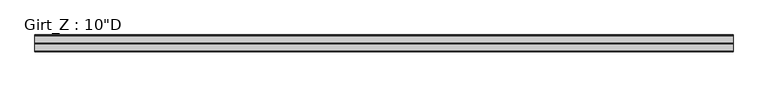
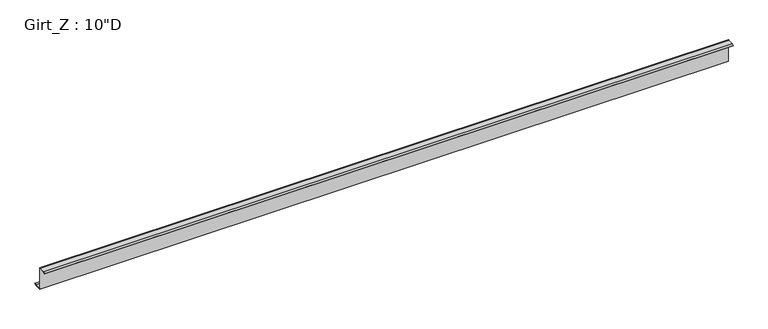
"""IFC4 building model written with IfcOpenShell, lengths in millimetres: beam geometry."""

from ifc_helpers import new_model, si_unit, point, frame, frame_2d, origin, place, context, project, spatial, polyline, circle_curve, trimmed, segment, composite_curve, outline, extrude, source, transform, mapped, element, save


def beam_e7052807(model_context):
    return source(origin(), model_context, "Body", "SweptSolid", [
        extrude(outline(composite_curve([segment(polyline([(-77.9859375, 127.0), (-3.3734375, 127.0)]), True, "CONTINUOUS"), segment(trimmed(circle_curve(frame_2d((-3.3734375, 122.2375)), 4.7625), [point((-3.3734375, 127.0))], [point((1.3890625, 122.2375))], False, "CARTESIAN"), True, "CONTINUOUS"), segment(polyline([(1.3890625, 122.2375), (1.3890625, -122.2389339)]), True, "CONTINUOUS"), segment(trimmed(circle_curve(frame_2d((3.3748024, -122.2389339)), 1.9857399), [point((1.3890625, -122.2389339))], [point((3.2694106, -124.221875))], True, "CARTESIAN"), True, "CONTINUOUS"), segment(polyline([(3.2694106, -124.221875), (83.0404765, -124.221875), (94.4528742, -110.621109), (96.5810415, -112.4068534), (84.3359375, -127.0), (-1.3890625, -127.0), (-1.3890625, 122.2381931)]), True, "CONTINUOUS"), segment(trimmed(circle_curve(frame_2d((-3.3741066, 122.2381931)), 1.9850441), [point((-1.3890625, 122.2381931))], [point((-3.3005807, 124.221875))], True, "CARTESIAN"), True, "CONTINUOUS"), segment(polyline([(-3.3005807, 124.221875), (-76.6904765, 124.221875), (-88.1028742, 110.621109), (-90.2310415, 112.4068534), (-77.9859375, 127.0)]), True, "CONTINUOUS")], self_intersect=False)), frame((-3811.1049, 0.0, 0.0), z_axis=(1.0, 0.0, 0.0), x_axis=(0.0, 1.0, 0.0)), (0.0, 0.0, 1.0), 7692.644),
    ])


if __name__ == "__main__":
    model = new_model("IFC4")
    model_context = context("Model", 3, world=origin())
    ifc_project = project(units=[si_unit("LENGTHUNIT", "METRE", prefix="MILLI")], contexts=[model_context])
    site = spatial("IfcSite", under=ifc_project)
    building = spatial("IfcBuilding", under=site)
    placement = place(None, origin())
    beam_shape = beam_e7052807(model_context)
    element("IfcBeam", 1, ObjectType="Girt_Z : 10\"D", at=placement, inside=building, context=model_context, shape_type="MappedRepresentation", body=[
        mapped(beam_shape, transform((0.0, 0.0, 0.0), x_axis=(1.0, 0.0, 0.0), y_axis=(0.0, 1.0, 0.0), z_axis=(0.0, 0.0, 1.0))),
    ])
    save(model, "model.ifc")

# Revit data of these elements
# Type "Girt_Z : 10\"D"
#   half leg = 0' - 1 11/16"
#   Web_Thickness = 0' - 0 7/64"
#   Length [instance default] = 10' - 0"
#   Leg_2 = 0' - 3 3/8"
#   Leg_1 = 0' - 3 1/8"
#   Height = 0' - 10"
#   Structural Material [instance default] = none
